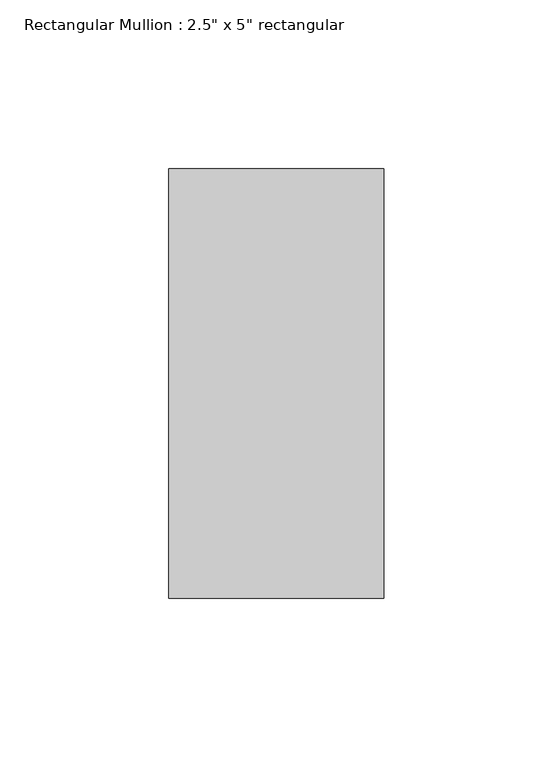
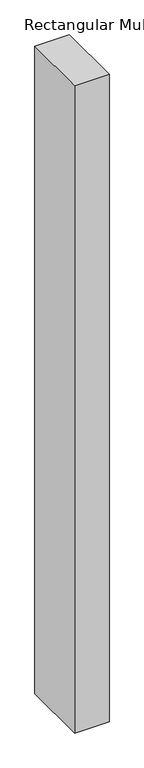
"""IFC4 building model written with IfcOpenShell, lengths in millimetres: member geometry."""

from ifc_helpers import new_model, si_unit, frame, origin, place, context, project, spatial, polyline, outline, extrude, source, transform, mapped, element, save


def member_e7b2e991(model_context):
    return source(origin(), model_context, "Body", "SweptSolid", [
        extrude(outline(polyline([(0.0, 63.5), (0.0, -63.5), (-63.5, -63.5), (-63.5, 63.5), (0.0, 63.5)])), frame((0.0, 0.0, -1263.65), z_axis=(0.0, 0.0, 1.0), x_axis=(1.0, 0.0, 0.0)), (0.0, 0.0, 1.0), 1263.65),
    ])


if __name__ == "__main__":
    model = new_model("IFC4")
    model_context = context("Model", 3, world=origin())
    ifc_project = project(units=[si_unit("LENGTHUNIT", "METRE", prefix="MILLI")], contexts=[model_context])
    site = spatial("IfcSite", under=ifc_project)
    building = spatial("IfcBuilding", under=site)
    placement = place(None, origin())
    member_shape = member_e7b2e991(model_context)
    element("IfcMember", 1, ObjectType="Rectangular Mullion : 2.5\" x 5\" rectangular", at=placement, inside=building, context=model_context, shape_type="MappedRepresentation", body=[
        mapped(member_shape, transform((0.0, 0.0, 0.0), x_axis=(1.0, 0.0, 0.0), y_axis=(0.0, 1.0, 0.0), z_axis=(0.0, 0.0, 1.0))),
    ])
    save(model, "model.ifc")

# Revit data of these elements
# Type "Rectangular Mullion : 2.5\" x 5\" rectangular"
#   built-in parameter 1007304 = 0.416667 (stored number, unit not read)
#   built-in parameter 1007301 = 0.104167 (stored number, unit not read)
#   built-in parameter 1007300 = 0.104167 (stored number, unit not read)
# Element 1 (IfcMember, "Rectangular Mullion : 2.5\" x 5\" rectangular")
#   Materials on its faces: "Metal - Aluminum"
# Materials
#   "Metal - Aluminum": class "Metal", colour RGB 140 140 140, transparency 0
